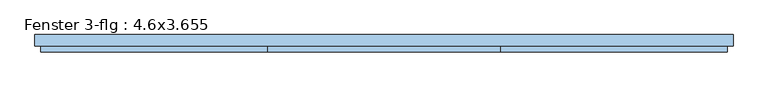
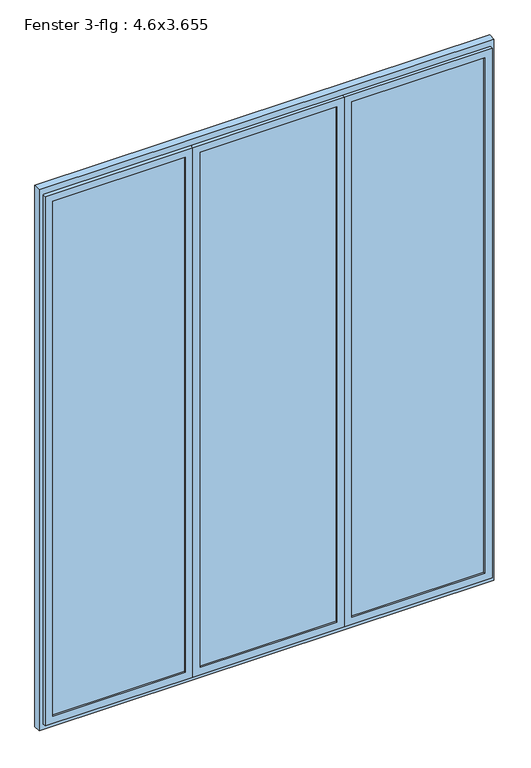
"""IFC4 building model written with IfcOpenShell, lengths in millimetres: window geometry, Fenster 3-flg : 4.6x3.655."""

from ifc_helpers import new_model, si_unit, frame, origin, place, context, project, spatial, polyline, outline, extrude, faceted_brep, source, transform, mapped, element, save


def fenster_3_flg_4_6x3_655_56bec587(model_context):
    return source(origin(), model_context, "Body", "SolidModel", [
        extrude(outline(polyline([(1336.6666667, 45.0), (1336.6666667, -15.0), (1276.6666667, -15.0), (1276.6666667, 45.0), (1336.6666667, 45.0)])), frame((0.0, 0.0, 1080.0), z_axis=(0.0, 0.0, 1.0), x_axis=(1.0, 0.0, 0.0)), (0.0, 0.0, 1.0), 4440.0),
        extrude(outline(polyline([(118.3333333, 45.0), (118.3333333, -15.0), (58.3333333, -15.0), (58.3333333, 45.0), (118.3333333, 45.0)])), frame((0.0, 0.0, 1080.0), z_axis=(0.0, 0.0, 1.0), x_axis=(1.0, 0.0, 0.0)), (0.0, 0.0, 1.0), 4440.0),
        extrude(outline(polyline([(5600.0, 2525.0), (5600.0, -1130.0), (1000.0, -1130.0), (1000.0, 2525.0), (5600.0, 2525.0)]), holes=[polyline([(5520.0, 2465.0), (1080.0, 2465.0), (1080.0, -1070.0), (5520.0, -1070.0), (5520.0, 2465.0)])]), frame((0.0, -15.0, 0.0), z_axis=(0.0, 1.0, 0.0), x_axis=(0.0, 0.0, 1.0)), (0.0, 0.0, 1.0), 60.0),
        faceted_brep([(1306.6666667, -15.0, 5550.0), (1306.6666667, -45.0, 5550.0), (1306.6666667, -45.0, 1050.0), (1306.6666667, -15.0, 1050.0), (88.3333333, -45.0, 5550.0), (88.3333333, -45.0, 1050.0), (1246.6666667, -45.0, 1110.0), (148.3333333, -45.0, 1110.0), (148.3333333, -45.0, 5490.0), (1246.6666667, -45.0, 5490.0), (88.3333333, -15.0, 1050.0), (88.3333333, -15.0, 5550.0), (1276.6666667, -15.0, 5520.0), (118.3333333, -15.0, 5520.0), (118.3333333, -15.0, 1080.0), (1276.6666667, -15.0, 1080.0), (1276.6666667, 15.0, 5520.0), (1276.6666667, 15.0, 1080.0), (118.3333333, 15.0, 1080.0), (118.3333333, 15.0, 5520.0), (1246.6666667, 15.0, 5490.0), (148.3333333, 15.0, 5490.0), (148.3333333, 15.0, 1110.0), (1246.6666667, 15.0, 1110.0)], [[[0, 1, 2, 3]], [[1, 4, 5, 2], [6, 7, 8, 9]], [[3, 2, 5, 10]], [[3, 10, 11, 0], [12, 13, 14, 15]], [[16, 12, 15, 17]], [[17, 15, 14, 18]], [[17, 18, 19, 16], [20, 21, 22, 23]], [[9, 20, 23, 6]], [[6, 23, 22, 7]], [[10, 5, 4, 11]], [[18, 14, 13, 19]], [[7, 22, 21, 8]], [[11, 4, 1, 0]], [[19, 13, 12, 16]], [[8, 21, 20, 9]]]),
        faceted_brep([(88.3333333, -15.0, 5550.0), (88.3333333, -45.0, 5550.0), (88.3333333, -45.0, 1050.0), (88.3333333, -15.0, 1050.0), (-1100.0, -45.0, 5550.0), (-1100.0, -45.0, 1050.0), (28.3333333, -45.0, 1110.0), (-1040.0, -45.0, 1110.0), (-1040.0, -45.0, 5490.0), (28.3333333, -45.0, 5490.0), (-1100.0, -15.0, 1050.0), (-1100.0, -15.0, 5550.0), (58.3333333, -15.0, 5520.0), (-1070.0, -15.0, 5520.0), (-1070.0, -15.0, 1080.0), (58.3333333, -15.0, 1080.0), (58.3333333, 15.0, 5520.0), (58.3333333, 15.0, 1080.0), (-1070.0, 15.0, 1080.0), (-1070.0, 15.0, 5520.0), (28.3333333, 15.0, 5490.0), (-1040.0, 15.0, 5490.0), (-1040.0, 15.0, 1110.0), (28.3333333, 15.0, 1110.0)], [[[0, 1, 2, 3]], [[1, 4, 5, 2], [6, 7, 8, 9]], [[3, 2, 5, 10]], [[3, 10, 11, 0], [12, 13, 14, 15]], [[16, 12, 15, 17]], [[17, 15, 14, 18]], [[17, 18, 19, 16], [20, 21, 22, 23]], [[9, 20, 23, 6]], [[6, 23, 22, 7]], [[10, 5, 4, 11]], [[18, 14, 13, 19]], [[7, 22, 21, 8]], [[11, 4, 1, 0]], [[19, 13, 12, 16]], [[8, 21, 20, 9]]]),
        faceted_brep([(2495.0, -15.0, 5550.0), (2495.0, -45.0, 5550.0), (2495.0, -45.0, 1050.0), (2495.0, -15.0, 1050.0), (1306.6666667, -45.0, 5550.0), (1306.6666667, -45.0, 1050.0), (2435.0, -45.0, 1110.0), (1366.6666667, -45.0, 1110.0), (1366.6666667, -45.0, 5490.0), (2435.0, -45.0, 5490.0), (1306.6666667, -15.0, 1050.0), (1306.6666667, -15.0, 5550.0), (2465.0, -15.0, 5520.0), (1336.6666667, -15.0, 5520.0), (1336.6666667, -15.0, 1080.0), (2465.0, -15.0, 1080.0), (2465.0, 15.0, 5520.0), (2465.0, 15.0, 1080.0), (1336.6666667, 15.0, 1080.0), (1336.6666667, 15.0, 5520.0), (2435.0, 15.0, 5490.0), (1366.6666667, 15.0, 5490.0), (1366.6666667, 15.0, 1110.0), (2435.0, 15.0, 1110.0)], [[[0, 1, 2, 3]], [[1, 4, 5, 2], [6, 7, 8, 9]], [[3, 2, 5, 10]], [[3, 10, 11, 0], [12, 13, 14, 15]], [[16, 12, 15, 17]], [[17, 15, 14, 18]], [[17, 18, 19, 16], [20, 21, 22, 23]], [[9, 20, 23, 6]], [[6, 23, 22, 7]], [[10, 5, 4, 11]], [[18, 14, 13, 19]], [[7, 22, 21, 8]], [[11, 4, 1, 0]], [[19, 13, 12, 16]], [[8, 21, 20, 9]]]),
        extrude(outline(polyline([(2435.0, -30.0), (1366.6666667, -30.0), (1366.6666667, 0.0), (2435.0, 0.0), (2435.0, -30.0)])), frame((0.0, 0.0, 1110.0), z_axis=(0.0, 0.0, 1.0), x_axis=(1.0, 0.0, 0.0)), (0.0, 0.0, 1.0), 4380.0),
        extrude(outline(polyline([(1246.6666667, -30.0), (148.3333333, -30.0), (148.3333333, 0.0), (1246.6666667, 0.0), (1246.6666667, -30.0)])), frame((0.0, 0.0, 1110.0), z_axis=(0.0, 0.0, 1.0), x_axis=(1.0, 0.0, 0.0)), (0.0, 0.0, 1.0), 4380.0),
        extrude(outline(polyline([(28.3333333, -30.0), (-1040.0, -30.0), (-1040.0, 0.0), (28.3333333, 0.0), (28.3333333, -30.0)])), frame((0.0, 0.0, 1110.0), z_axis=(0.0, 0.0, 1.0), x_axis=(1.0, 0.0, 0.0)), (0.0, 0.0, 1.0), 4380.0),
    ])


if __name__ == "__main__":
    model = new_model("IFC4")
    model_context = context("Model", 3, world=origin())
    ifc_project = project(units=[si_unit("LENGTHUNIT", "METRE", prefix="MILLI")], contexts=[model_context])
    site = spatial("IfcSite", under=ifc_project)
    building = spatial("IfcBuilding", under=site)
    placement = place(None, origin())
    fenster_3_flg_4_6x3_655_shape = fenster_3_flg_4_6x3_655_56bec587(model_context)
    element("IfcWindow", 1, ObjectType="Fenster 3-flg : 4.6x3.655", at=placement, inside=building, context=model_context, shape_type="MappedRepresentation", body=[
        mapped(fenster_3_flg_4_6x3_655_shape, transform((0.0, 0.0, 0.0), x_axis=(1.0, 0.0, 0.0), y_axis=(0.0, 1.0, 0.0), z_axis=(0.0, 0.0, 1.0))),
    ])
    save(model, "model.ifc")

# Revit data of these elements
# Type "Fenster 3-flg : 4.6x3.655"
#   Type Mark = "80"
#   Operation = "TriplePanelVertical"
#   Keynote = "16.05.01"
#   Visual Light Transmittance = 0.9
#   Solar Heat Gain Coefficient = 0.78
#   Rough Height = 4.600 m
#   Rough Width = 3.655 m
#   Heat Transfer Coefficient (U) = 3.6886 W/(m²·K)
#   Rahmentiefe = 0.060 m
#   Breite unterer Rahmen = 0.080 m
#   Breite oberer  Rahmen = 0.080 m
#   Rahmenbreite = 0.060 m
#   Height = 4.600 m
#   Tiefe Flügel = 0.060 m
#   Flügelbreite = 0.060 m
#   Einbautiefe (von außen) [instance default] = 0.080 m
#   Width = 3.655 m
#   Bild [instance default] = none
#   Glas [instance default] = none
#   Fensterflügel [instance default] = none
#   Innere Fensterbank [instance default] = none
#   Äußere Fensterbank [instance default] = none
#   Construction Type Id = ""
#   Wall Closure = (empty or 0)
#   Analytic Construction = (empty or 0)
# Element 1 (IfcWindow, "Fenster 3-flg : 4.6x3.655")
#   Einbautiefe (von außen) = 0.230 m
#   Materials on its faces: "Kunststoff - Weiß", "Glas"
# Materials
#   "Kunststoff - Weiß": class "Kunststoff", colour RGB 249 249 249, transparency 0, Cost = 0
#   "Glas": class "Glas", colour RGB 0 0 255, transparency 0.75, Comments = "Render-Darstellung nicht aktualisiert ", Cost = 0
